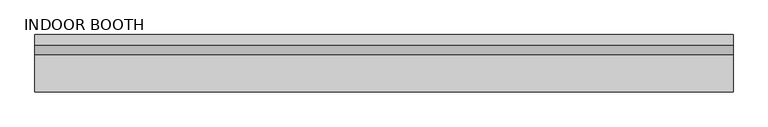
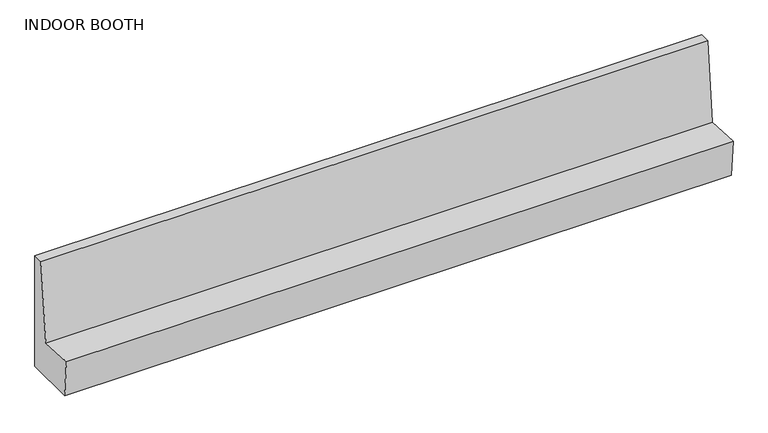
"""IFC4 building model written with IfcOpenShell, lengths in millimetres: furniture geometry, OD_CW_Booth : INDOOR BOOTH."""

import ifcopenshell
import ifcopenshell.guid

model = None  # the IFC model being written
_history = None  # IfcOwnerHistory: only IFC2X3 demands one
_inside = {}  # id of a spatial element -> (the spatial element, [elements in it])
_under = {}  # id of a project, library or spatial element -> (it, [spatial elements below it])
_declared = {}  # id of a project -> (the project, [libraries it declares])
_typed = {}  # id of a type object -> (the type object, [elements of that type])
_made_of = {}  # id of a material, layer set ... -> (it, [elements and type objects made of it])


def new_model(schema):
    """Start an empty IFC model of exactly this schema.

    Asked for "IFC4X3", IfcOpenShell would pick the latest addendum, in which some entities
    have other attributes; the version numbers below select the first issue.
    IFC2X3 requires an IfcOwnerHistory on every rooted entity: one is made here for all.
    """
    global model, _history
    if schema == "IFC4X3":
        model = ifcopenshell.file(schema_version=(4, 3, 0, 0))
    else:
        model = ifcopenshell.file(schema=schema)
    _inside.clear()
    _under.clear()
    _declared.clear()
    _typed.clear()
    _made_of.clear()
    _history = None
    if model.schema == "IFC2X3":
        org = make("IfcOrganization", Name="unknown")
        user = make(
            "IfcPersonAndOrganization",
            ThePerson=make("IfcPerson", FamilyName="unknown"),
            TheOrganization=org,
        )
        app = make(
            "IfcApplication",
            ApplicationDeveloper=org,
            Version="unknown",
            ApplicationFullName="unknown",
            ApplicationIdentifier="unknown",
        )
        _history = make(
            "IfcOwnerHistory",
            OwningUser=user,
            OwningApplication=app,
            ChangeAction="ADDED",
            CreationDate=0,
        )
    return model


def make(cls, **values):
    """One entity of the class cls with the attributes given. An attribute that is None is left unset."""
    return model.create_entity(
        cls, **{name: value for name, value in values.items() if value is not None}
    )


def rooted(cls, **values):
    """An entity with a GlobalId (a new one), such as an element, a storey or a relation."""
    return make(cls, GlobalId=ifcopenshell.guid.new(), OwnerHistory=_history, **values)


def si_unit(unit_type, name, prefix=None):
    """IfcSIUnit, for example si_unit("LENGTHUNIT", "METRE", prefix="MILLI")."""
    return make("IfcSIUnit", UnitType=unit_type, Prefix=prefix, Name=name)


def assignment(units):
    """IfcUnitAssignment: the units of a project."""
    return None if units is None else make("IfcUnitAssignment", Units=units)


def point(xyz):
    """IfcCartesianPoint."""
    return None if xyz is None else make("IfcCartesianPoint", Coordinates=xyz)


def direction(xyz):
    """IfcDirection."""
    return None if xyz is None else make("IfcDirection", DirectionRatios=xyz)


def frame(location, z_axis=None, x_axis=None):
    """IfcAxis2Placement3D, a coordinate frame: its origin and axes. An axis left out is left unset."""
    return make(
        "IfcAxis2Placement3D",
        Location=point(location),
        Axis=direction(z_axis),
        RefDirection=direction(x_axis),
    )


def origin():
    """The frame at (0, 0, 0) with its axes left unset."""
    return frame((0.0, 0.0, 0.0))


def place(relative_to, where):
    """IfcLocalPlacement: puts the frame where relative to a parent placement (None: the world)."""
    return make(
        "IfcLocalPlacement", PlacementRelTo=relative_to, RelativePlacement=where
    )


def context(
    kind, dimensions, precision=None, world=None, true_north=None, identifier=None
):
    """IfcGeometricRepresentationContext, for example the 3D "Model" context."""
    return make(
        "IfcGeometricRepresentationContext",
        ContextIdentifier=identifier,
        ContextType=kind,
        CoordinateSpaceDimension=dimensions,
        Precision=precision,
        WorldCoordinateSystem=world,
        TrueNorth=true_north,
    )


def project(units=None, contexts=None):
    """IfcProject with its units and contexts."""
    return rooted(
        "IfcProject",
        Name="project",
        RepresentationContexts=contexts,
        UnitsInContext=assignment(units),
    )


def spatial(cls, under=None, at=None, **own):
    """A site, building, storey or space (cls), placed at a placement, below another one or the project."""
    s = rooted(cls, ObjectPlacement=at, **own)
    if under is not None:
        _under.setdefault(under.id(), (under, []))[1].append(s)
    return s


def polyline(points):
    """IfcPolyline through the points."""
    return make("IfcPolyline", Points=[point(p) for p in points])


def outline(outer, holes=None, kind="AREA"):
    """IfcArbitraryClosedProfileDef: a profile drawn as a closed curve; with holes, ...WithVoids."""
    if holes is None:
        return make("IfcArbitraryClosedProfileDef", ProfileType=kind, OuterCurve=outer)
    return make(
        "IfcArbitraryProfileDefWithVoids",
        ProfileType=kind,
        OuterCurve=outer,
        InnerCurves=holes,
    )


def extrude(swept, where, along, depth):
    """IfcExtrudedAreaSolid: the profile swept, set in the frame where, extruded along a direction by depth."""
    return make(
        "IfcExtrudedAreaSolid",
        SweptArea=swept,
        Position=where,
        ExtrudedDirection=direction(along),
        Depth=depth,
    )


def shape(context_of_items, identifier, shape_type, items):
    """IfcShapeRepresentation: the items that make up one representation, for example the "Body"."""
    return make(
        "IfcShapeRepresentation",
        ContextOfItems=context_of_items,
        RepresentationIdentifier=identifier,
        RepresentationType=shape_type,
        Items=items,
    )


def source(mapping_origin, context_of_items, identifier, shape_type, items):
    """IfcRepresentationMap: a shape defined once, which mapped items show again and again."""
    return make(
        "IfcRepresentationMap",
        MappingOrigin=mapping_origin,
        MappedRepresentation=shape(context_of_items, identifier, shape_type, items),
    )


def transform(
    local_origin,
    x_axis=None,
    y_axis=None,
    z_axis=None,
    scale=None,
    scale2=None,
    scale3=None,
    uniform=True,
):
    """IfcCartesianTransformationOperator3D, or its non-uniform kind. x_axis, y_axis, z_axis: its Axis1, 2, 3."""
    if uniform:
        return make(
            "IfcCartesianTransformationOperator3D",
            Axis1=direction(x_axis),
            Axis2=direction(y_axis),
            LocalOrigin=point(local_origin),
            Scale=scale,
            Axis3=direction(z_axis),
        )
    return make(
        "IfcCartesianTransformationOperator3DnonUniform",
        Axis1=direction(x_axis),
        Axis2=direction(y_axis),
        LocalOrigin=point(local_origin),
        Scale=scale,
        Axis3=direction(z_axis),
        Scale2=scale2,
        Scale3=scale3,
    )


def mapped(mapping_source, mapping_target):
    """IfcMappedItem: shows the shape of a source again, moved by a transform."""
    return make(
        "IfcMappedItem", MappingSource=mapping_source, MappingTarget=mapping_target
    )


def made_of(thing, what):
    """Note that an element or type object is made of a material, layer set ...; save() writes the relation."""
    if what is not None:
        _made_of.setdefault(what.id(), (what, []))[1].append(thing)
    return thing


def element(
    cls,
    number,
    at=None,
    inside=None,
    cuts=None,
    type_object=None,
    material=None,
    context=None,
    identifier="Body",
    shape_type=None,
    held_by="IfcProductDefinitionShape",
    body=None,
    shapes=None,
    **own,
):
    """One element of the class cls, such as IfcWall. Its Tag is "e" and its number.

    at: its placement. inside: the storey or other place that contains it. cuts: it is an
    opening in that element (IfcRelVoidsElement). A single representation is given by context,
    identifier, shape_type and body (its items); several are given by shapes. held_by: the class
    of the entity that holds the representations. save() writes the other relations.
    """
    e = rooted(cls, Tag="e%d" % number, ObjectPlacement=at, **own)
    if body is not None:
        shapes = [shape(context, identifier, shape_type, body)]
    if shapes is not None:
        e.Representation = make(held_by, Representations=shapes)
    if inside is not None:
        _inside.setdefault(inside.id(), (inside, []))[1].append(e)
    if cuts is not None:
        rooted(
            "IfcRelVoidsElement", RelatingBuildingElement=cuts, RelatedOpeningElement=e
        )
    if type_object is not None:
        _typed.setdefault(type_object.id(), (type_object, []))[1].append(e)
    return made_of(e, material)


def aggregate(whole, parts):
    """IfcRelAggregates: a whole, such as a stair, and the parts it consists of."""
    return rooted("IfcRelAggregates", RelatingObject=whole, RelatedObjects=parts)


def save(model, path):
    """Write the relations noted so far, then the file.

    IfcRelAggregates (storeys below a building ...), IfcRelContainedInSpatialStructure (elements
    in a storey), IfcRelDefinesByType, IfcRelAssociatesMaterial and IfcRelDeclares: one each for
    every whole, place, type object, material and project.
    """
    for whole, parts in _under.values():
        aggregate(whole, parts)
    for where, things in _inside.values():
        rooted(
            "IfcRelContainedInSpatialStructure",
            RelatedElements=things,
            RelatingStructure=where,
        )
    for kind, things in _typed.values():
        rooted("IfcRelDefinesByType", RelatedObjects=things, RelatingType=kind)
    for what, things in _made_of.values():
        rooted("IfcRelAssociatesMaterial", RelatedObjects=things, RelatingMaterial=what)
    for by, libraries in _declared.values():
        rooted("IfcRelDeclares", RelatingContext=by, RelatedDefinitions=libraries)
    model.write(path)


def indoor_booth_d0ba213d(model_context):
    return source(origin(), model_context, "Body", "SweptSolid", [
        extrude(outline(polyline([(609.6, 1397.0), (609.6, 0.0), (-3.4100193, 0.0), (-43.0849153, 453.4861359), (382.9385128, 431.1591941), (484.4524721, 1397.0), (609.6, 1397.0)])), frame((18.7377049, 0.0, 0.0), z_axis=(1.0, 0.0, 0.0), x_axis=(0.0, 1.0, 0.0)), (0.0, 0.0, 1.0), 7958.479089),
    ])


if __name__ == "__main__":
    model = new_model("IFC4")
    model_context = context("Model", 3, world=origin())
    ifc_project = project(units=[si_unit("LENGTHUNIT", "METRE", prefix="MILLI")], contexts=[model_context])
    site = spatial("IfcSite", under=ifc_project)
    building = spatial("IfcBuilding", under=site)
    placement = place(None, origin())
    indoor_booth_shape = indoor_booth_d0ba213d(model_context)
    element("IfcFurniture", 1, ObjectType="OD_CW_Booth : INDOOR BOOTH", at=placement, inside=building, context=model_context, shape_type="MappedRepresentation", body=[
        mapped(indoor_booth_shape, transform((0.0, 0.0, 0.0), x_axis=(1.0, 0.0, 0.0), y_axis=(0.0, 1.0, 0.0), z_axis=(0.0, 0.0, 1.0))),
    ])
    save(model, "model.ifc")

# Revit data of these elements
# Type "OD_CW_Booth : INDOOR BOOTH"
#   Type Mark = "TYPE-INDOOR"
#   Width = 4' - 0"
#   OD_CW_Width [instance default] = 2' - 10"
#   OD_CW_Length [instance default] = 26' - 1 83/256"
#   OD_CW_Height [instance default] = 2' - 3"
#   Height = 3' - 0"
#   Depth = 2' - 0"
#   Seating Count [instance default] = 10
#   Seating Count [instance default] = 10
#   OD_CW_Material_Front Panel [instance default] = none
#   OD_CW_Material_Body [instance default] = none
# Element 1 (IfcFurniture, "OD_CW_Booth : INDOOR BOOTH")
#   OD_CW_Length = 26' - 1.32595"
#   OD_CW_Material_Body = Sals Wood
#   Materials on its faces: "Sals Wood"
# Materials
#   "Sals Wood": class "Wood", colour RGB 198 202 183, transparency 0, Description = "Generic wood", Cost = 0
